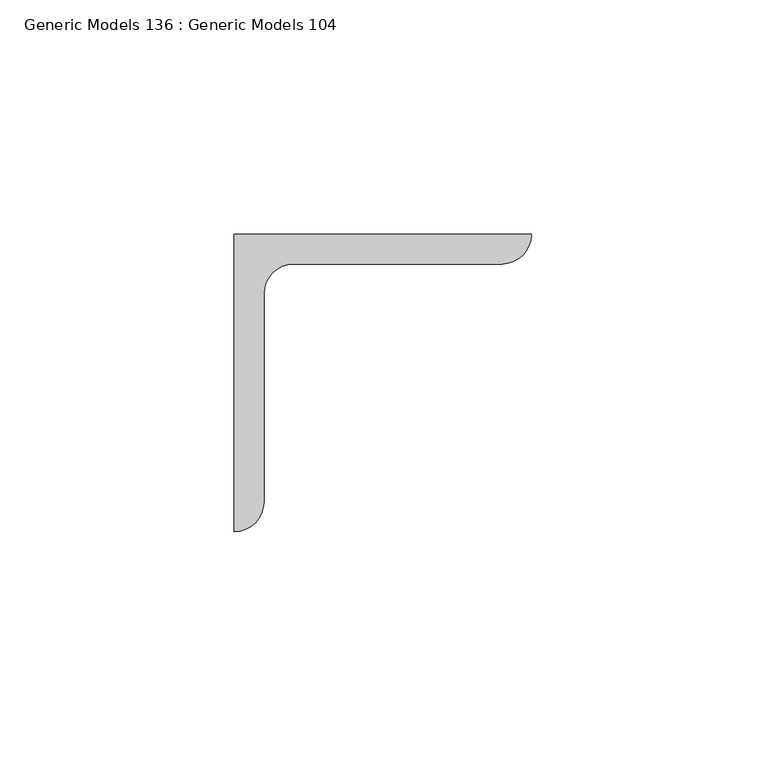
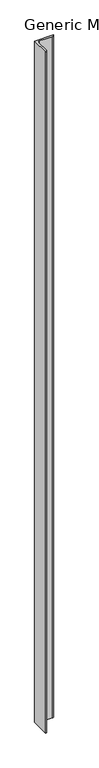
"""IFC4 building model written with IfcOpenShell, lengths in millimetres: proxy geometry, Generic Models 136 : Generic Models 104."""

from ifc_helpers import new_model, si_unit, point, frame, frame_2d, origin, place, context, project, spatial, polyline, circle_curve, trimmed, segment, composite_curve, outline, extrude, source, transform, mapped, element, save


def generic_models_136_generic_models_104_c3016f2e(model_context):
    return source(origin(), model_context, "Body", "SweptSolid", [
        extrude(outline(composite_curve([segment(polyline([(29176.0240778, 41071.1196612), (29239.5240778, 41071.1196612)]), True, "CONTINUOUS"), segment(trimmed(circle_curve(frame_2d((29233.1740778, 41071.1196612)), 6.35), [point((29239.5240778, 41071.1196612))], [point((29233.1740778, 41064.7696612))], False, "CARTESIAN"), True, "CONTINUOUS"), segment(polyline([(29233.1740778, 41064.7696612), (29188.7240778, 41064.7696612)]), True, "CONTINUOUS"), segment(trimmed(circle_curve(frame_2d((29188.7240778, 41058.4196612)), 6.35), [point((29188.7240778, 41064.7696612))], [point((29182.3740778, 41058.4196612))], True, "CARTESIAN"), True, "CONTINUOUS"), segment(polyline([(29182.3740778, 41058.4196612), (29182.3740778, 41013.9696612)]), True, "CONTINUOUS"), segment(trimmed(circle_curve(frame_2d((29176.0240778, 41013.9696612)), 6.35), [point((29182.3740778, 41013.9696612))], [point((29176.0240778, 41007.6196612))], False, "CARTESIAN"), True, "CONTINUOUS"), segment(polyline([(29176.0240778, 41007.6196612), (29176.0240778, 41071.1196612)]), True, "CONTINUOUS")], self_intersect=False)), frame((0.0, 0.0, 266407.9), z_axis=(0.0, 0.0, 1.0), x_axis=(1.0, 0.0, 0.0)), (0.0, 0.0, 1.0), 2432.1044757),
    ])


if __name__ == "__main__":
    model = new_model("IFC4")
    model_context = context("Model", 3, world=origin())
    ifc_project = project(units=[si_unit("LENGTHUNIT", "METRE", prefix="MILLI")], contexts=[model_context])
    site = spatial("IfcSite", under=ifc_project)
    building = spatial("IfcBuilding", under=site)
    placement = place(None, origin())
    generic_models_136_generic_models_104_shape = generic_models_136_generic_models_104_c3016f2e(model_context)
    element("IfcBuildingElementProxy", 1, Name="Generic Models 136 : Generic Models 104", ObjectType="Generic Models 136 : Generic Models 104", at=placement, inside=building, context=model_context, shape_type="MappedRepresentation", body=[
        mapped(generic_models_136_generic_models_104_shape, transform((0.0, 0.0, 0.0), x_axis=(1.0, 0.0, 0.0), y_axis=(0.0, 1.0, 0.0), z_axis=(0.0, 0.0, 1.0))),
    ])
    save(model, "model.ifc")

# Revit data of these elements
# Element 1 (IfcBuildingElementProxy, "Generic Models 136 : Generic Models 104")
#   Materials on its faces: "(2) BACK/BACK GALVANIZED ANGLES (2) L2 1/2 X 2 1/2 X 1/4\")"
# Materials
#   "(2) BACK/BACK GALVANIZED ANGLES (2) L2 1/2 X 2 1/2 X 1/4\")": class "Unassigned", colour RGB 211 211 211, transparency 0, Cost = 0
